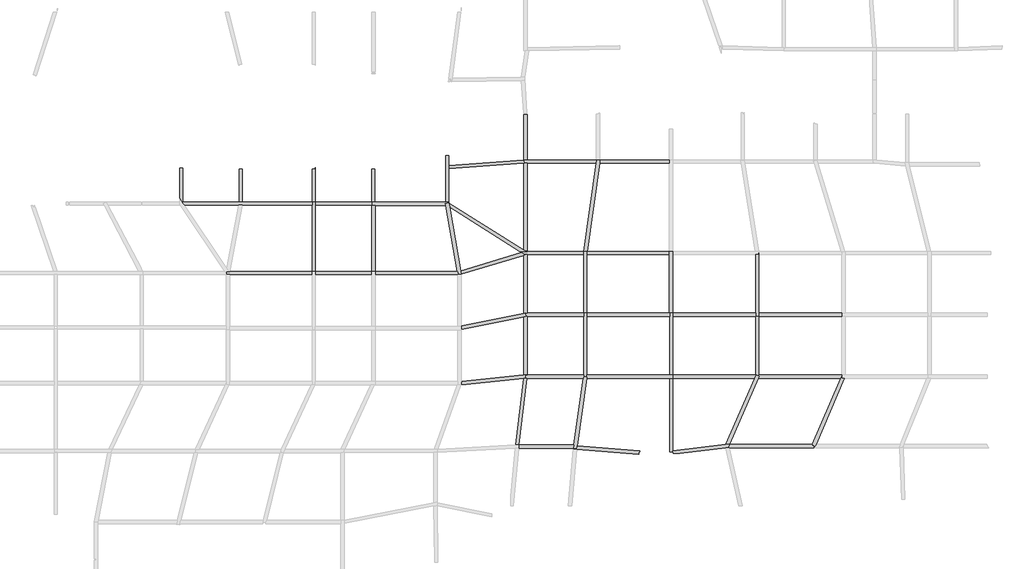
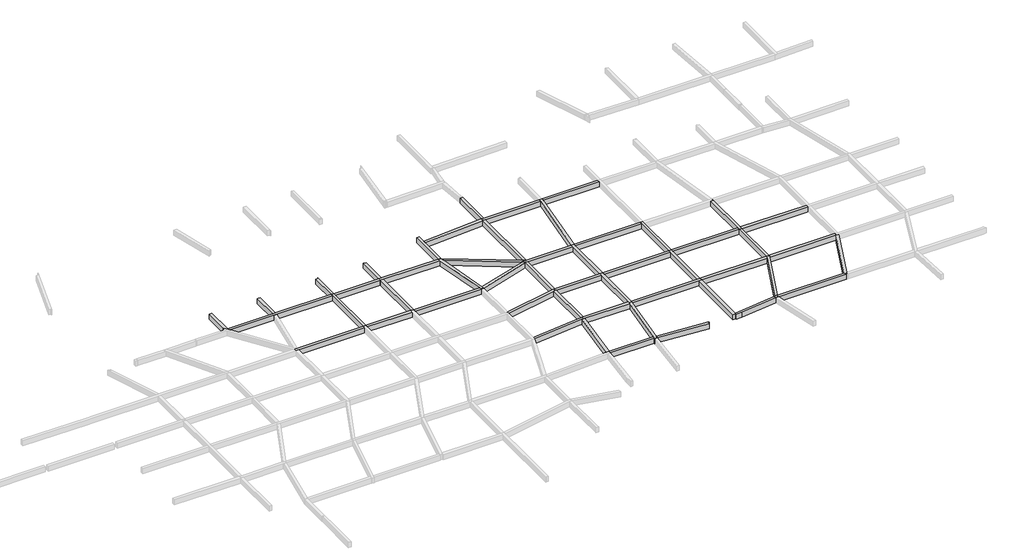
# One storey, part 10 of 15: 51 beams.
"""IFC4 building model written with IfcOpenShell, lengths in millimetres."""

from ifc_helpers import new_model, si_unit, frame, origin, place, context, project, spatial, polyline, outline, extrude, faceted_brep, element, save

model = new_model("IFC4")

# Units and contexts
model_context = context("Model", 3, world=origin())
ifc_project = project(units=[si_unit("LENGTHUNIT", "METRE", prefix="MILLI")], contexts=[model_context])

# Site, building, storey
site = spatial("IfcSite", under=ifc_project)
building = spatial("IfcBuilding", under=site)
storey = spatial("IfcBuildingStorey", under=building, Name="层高", Elevation=3300.0)

# Beams
placement = place(None, origin())
element("IfcBeam", 1, ObjectType="混凝土 - 矩形梁 : KL_beam", at=placement, inside=storey, context=model_context, shape_type="SweptSolid", body=[
    extrude(outline(polyline([(208450.3009381, 80084.9176514), (208450.3009381, 80384.9176514), (213550.3009381, 80384.9176514), (213550.3009381, 80084.9176514), (208450.3009381, 80084.9176514)])), frame((0.0, 0.0, 2700.0), z_axis=(0.0, 0.0, 1.0), x_axis=(1.0, 0.0, 0.0)), (0.0, 0.0, 1.0), 600.0),
])
element("IfcBeam", 2, ObjectType="混凝土 - 矩形梁 : KL_beam", at=placement, inside=storey, context=model_context, shape_type="Brep", body=[
    faceted_brep([(208150.3009381, 80092.1684205, 3300.0), (208150.3009381, 80384.9176514, 3300.0), (208450.3009381, 80384.9176514, 3300.0), (208450.3009381, 80392.1684205, 3300.0), (208150.3009381, 80392.1684205, 3300.0), (200691.8253203, 80392.1684205, 3300.0), (200590.9130323, 80392.1684205, 3300.0), (200361.325629, 80392.1684205, 3300.0), (200361.325629, 80196.1646357, 3300.0), (200361.325629, 80092.1684205, 3300.0), (200661.325629, 80092.1684205, 3300.0), (208150.3009381, 80092.1684205, 2700.0), (200361.325629, 80092.1684205, 2700.0), (200661.325629, 80092.1684205, 2700.0), (208150.3009381, 80384.9176514, 2700.0), (200361.325629, 80196.1646357, 2700.0), (200361.325629, 80392.1684205, 2700.0), (200590.9130323, 80392.1684205, 2700.0), (200691.8253203, 80392.1684205, 2700.0), (208150.3009381, 80392.1684205, 2700.0), (208450.3009381, 80392.1684205, 2700.0), (208450.3009381, 80384.9176514, 2700.0)], [[[0, 1, 2, 3, 4, 5, 6, 7, 8, 9, 10]], [[11, 0, 10, 9, 12, 13]], [[14, 11, 13, 12, 15, 16, 17, 18, 19, 20, 21]], [[16, 7, 6, 5, 4, 3, 20, 19, 18, 17]], [[14, 1, 0, 11]], [[1, 14, 21, 2]], [[9, 8, 7, 16, 15, 12]], [[20, 3, 2, 21]]]),
])
element("IfcBeam", 3, ObjectType="混凝土 - 矩形梁 : KL_beam", at=placement, inside=storey, context=model_context, shape_type="Brep", body=[
    faceted_brep([(232749.8021762, 70852.5016685, 3300.0), (233049.8021762, 70831.5236249, 3300.0), (233049.8021762, 70992.0126454, 3300.0), (233049.8021762, 76292.0126467, 3300.0), (233049.8021762, 76592.0126467, 3300.0), (232749.8021762, 76592.0126467, 3300.0), (232749.8021762, 76292.0126467, 3300.0), (232749.8021762, 70992.0126467, 3300.0), (233049.8021762, 70831.5236249, 2700.0), (233049.8021762, 70992.0126454, 2700.0), (233049.8021762, 76292.0126467, 2700.0), (233049.8021762, 76592.0126467, 2700.0), (232749.8021762, 70852.5016685, 2700.0), (232749.8021762, 70992.0126467, 2700.0), (232749.8021762, 76292.0126467, 2700.0), (232749.8021762, 76592.0126467, 2700.0)], [[[0, 1, 2, 3, 4, 5, 6, 7]], [[1, 8, 9, 10, 11, 4, 3, 2]], [[8, 12, 13, 14, 15, 11, 10, 9]], [[12, 0, 7, 6, 5, 15, 14, 13]], [[0, 12, 8, 1]], [[5, 4, 11, 15]]]),
])
element("IfcBeam", 4, ObjectType="混凝土 - 矩形梁 : KL_beam", at=placement, inside=storey, context=model_context, shape_type="Brep", body=[
    faceted_brep([(232124.0582724, 64244.513481, 3300.0), (232165.8855427, 64542.1299739, 3300.0), (233030.1951867, 70692.0126454, 3300.0), (233049.8021762, 70831.5236249, 3300.0), (232749.8021762, 70852.5016685, 3300.0), (232727.2469151, 70692.0126467, 3300.0), (231875.9120638, 64634.4504224, 3300.0), (231833.7498134, 64334.4504224, 3300.0), (231826.9778517, 64286.2654113, 3300.0), (232749.8021762, 70852.5016685, 2700.0), (232727.2469151, 70692.0126467, 2700.0), (231875.9120638, 64634.4504224, 2700.0), (231833.7498134, 64334.4504224, 2700.0), (231826.9778517, 64286.2654113, 2700.0), (233049.8021762, 70831.5236249, 2700.0), (233030.1951867, 70692.0126454, 2700.0), (232165.8855427, 64542.1299739, 2700.0), (232124.0582724, 64244.513481, 2700.0)], [[[0, 1, 2, 3, 4, 5, 6, 7, 8]], [[8, 7, 6, 5, 4, 9, 10, 11, 12, 13]], [[13, 12, 11, 10, 9, 14, 15, 16, 17]], [[3, 2, 1, 0, 17, 16, 15, 14]], [[3, 14, 9, 4]], [[0, 8, 13, 17]]]),
])
element("IfcBeam", 5, ObjectType="混凝土 - 矩形梁 : KL_beam", at=placement, inside=storey, context=model_context, shape_type="Brep", body=[
    faceted_brep([(233049.8021762, 70831.5236249, 3300.0), (233030.1951867, 70692.0126454, 3300.0), (240549.8021765, 70692.0126454, 3300.0), (240849.8021765, 70692.0126454, 3300.0), (240849.8021765, 70992.0126454, 3300.0), (240549.8021765, 70992.0126454, 3300.0), (233049.8021762, 70992.0126454, 3300.0), (240849.8021765, 70992.0126454, 2700.0), (240549.8021765, 70992.0126454, 2700.0), (233049.8021762, 70992.0126454, 2700.0), (233030.1951867, 70692.0126454, 2700.0), (233049.8021762, 70831.5236249, 2700.0), (240849.8021765, 70692.0126454, 2700.0), (240549.8021765, 70692.0126454, 2700.0)], [[[0, 1, 2, 3, 4, 5, 6]], [[4, 7, 8, 9, 6, 5]], [[10, 11, 9, 8, 7, 12, 13]], [[1, 10, 13, 12, 3, 2]], [[1, 0, 11, 10]], [[0, 6, 9, 11]], [[4, 3, 12, 7]]]),
])
element("IfcBeam", 6, ObjectType="混凝土 - 矩形梁 : KL_beam", at=placement, inside=storey, context=model_context, shape_type="Brep", body=[
    faceted_brep([(240849.8021765, 76592.0126467, 3300.0), (240838.5455997, 76592.0126467, 3300.0), (240549.8021765, 76592.0126467, 3300.0), (240549.8021765, 76292.0126467, 3300.0), (240549.8021765, 70992.0126454, 3300.0), (240849.8021765, 70992.0126454, 3300.0), (240849.8021765, 76302.5702379, 3300.0), (240849.8021765, 76592.0126467, 2700.0), (240849.8021765, 70992.0126454, 2700.0), (240849.8021765, 76302.5702379, 2700.0), (240549.8021765, 76592.0126467, 2700.0), (240838.5455997, 76592.0126467, 2700.0), (240549.8021765, 70992.0126454, 2700.0), (240549.8021765, 76292.0126467, 2700.0)], [[[0, 1, 2, 3, 4, 5, 6]], [[7, 0, 6, 5, 8, 9]], [[10, 11, 7, 9, 8, 12, 13]], [[2, 10, 13, 12, 4, 3]], [[5, 4, 12, 8]], [[2, 1, 0, 7, 11, 10]]]),
])
element("IfcBeam", 7, ObjectType="混凝土 - 矩形梁 : KL_beam", at=placement, inside=storey, context=model_context, shape_type="Brep", body=[
    faceted_brep([(233049.8021762, 76592.0126467, 3300.0), (233049.8021762, 76292.0126467, 3300.0), (240549.8021765, 76292.0126467, 3300.0), (240549.8021765, 76592.0126467, 3300.0), (240538.5455997, 76592.0126467, 3300.0), (233049.8021762, 76292.0126467, 2700.0), (240549.8021765, 76292.0126467, 2700.0), (233049.8021762, 76592.0126467, 2700.0), (240538.5455997, 76592.0126467, 2700.0), (240549.8021765, 76592.0126467, 2700.0)], [[[0, 1, 2, 3, 4]], [[1, 5, 6, 2]], [[5, 7, 8, 9, 6]], [[7, 0, 4, 3, 9, 8]], [[1, 0, 7, 5]], [[3, 2, 6, 9]]]),
])
element("IfcBeam", 8, ObjectType="混凝土 - 矩形梁 : KL_beam", at=placement, inside=storey, context=model_context, shape_type="Brep", body=[
    faceted_brep([(240849.8021765, 70692.0126454, 3300.0), (240549.8021765, 70692.0126454, 3300.0), (240549.8021765, 64002.26105, 3300.0), (240849.8021765, 64002.26105, 3300.0), (240849.8021765, 64111.1304578, 3300.0), (240549.8021765, 70692.0126454, 2700.0), (240549.8021765, 64002.26105, 2700.0), (240849.8021765, 70692.0126454, 2700.0), (240849.8021765, 64111.1304578, 2700.0), (240849.8021765, 64002.26105, 2700.0)], [[[0, 1, 2, 3, 4]], [[1, 5, 6, 2]], [[5, 7, 8, 9, 6]], [[7, 0, 4, 3, 9, 8]], [[1, 0, 7, 5]], [[3, 2, 6, 9]]]),
])
element("IfcBeam", 9, ObjectType="混凝土 - 矩形梁 : KL_beam", at=placement, inside=storey, context=model_context, shape_type="Brep", body=[
    faceted_brep([(245852.6551201, 64403.2000817, 3300.0), (245978.7341491, 64692.0126465, 3300.0), (245991.7500654, 64721.8285502, 3300.0), (245646.5106834, 64680.8252113, 3300.0), (240849.8021765, 64111.1304578, 3300.0), (240849.8021765, 64002.26105, 3300.0), (240859.8021767, 64002.26105, 3300.0), (240859.8021767, 63882.26105, 3300.0), (241466.459407, 63882.26105, 3300.0), (245632.7131892, 64377.0780516, 3300.0), (245758.4592979, 64392.0126465, 3300.0), (240849.8021765, 64111.1304578, 2700.0), (245991.7500654, 64721.8285502, 2700.0), (245646.5106834, 64680.8252113, 2700.0), (245978.7341491, 64692.0126465, 2700.0), (245852.6551201, 64403.2000817, 2700.0), (245758.4592979, 64392.0126465, 2700.0), (245632.7131892, 64377.0780516, 2700.0), (241466.459407, 63882.26105, 2700.0), (240859.8021767, 63882.26105, 2700.0), (240859.8021767, 64002.26105, 2700.0), (240849.8021765, 64002.26105, 2700.0)], [[[0, 1, 2, 3, 4, 5, 6, 7, 8, 9, 10]], [[11, 4, 3, 2, 12, 13]], [[12, 14, 15, 16, 17, 18, 19, 20, 21, 11, 13]], [[15, 0, 10, 9, 8, 18, 17, 16]], [[4, 11, 21, 5]], [[2, 1, 0, 15, 14, 12]], [[20, 6, 5, 21]], [[6, 20, 19, 7]], [[18, 8, 7, 19]]]),
])
element("IfcBeam", 10, ObjectType="混凝土 - 矩形梁 : KL_beam", at=placement, inside=storey, context=model_context, shape_type="Brep", body=[
    faceted_brep([(248676.5575109, 70871.9879428, 3300.0), (248649.8021768, 70883.6677897, 3300.0), (248401.6137516, 70992.0126454, 3300.0), (248270.650929, 70692.0126454, 3300.0), (245646.5106834, 64680.8252113, 3300.0), (245991.7500654, 64721.8285502, 3300.0), (248597.990601, 70692.0126454, 3300.0), (248401.6137516, 70992.0126454, 2700.0), (248270.650929, 70692.0126454, 2700.0), (245646.5106834, 64680.8252113, 2700.0), (248649.8021768, 70883.6677897, 2700.0), (248676.5575109, 70871.9879428, 2700.0), (248597.990601, 70692.0126454, 2700.0), (245991.7500654, 64721.8285502, 2700.0)], [[[0, 1, 2, 3, 4, 5, 6]], [[2, 7, 8, 9, 4, 3]], [[7, 10, 11, 12, 13, 9, 8]], [[11, 0, 6, 5, 13, 12]], [[5, 4, 9, 13]], [[0, 11, 10, 7, 2, 1]]]),
])
element("IfcBeam", 11, ObjectType="混凝土 - 矩形梁 : KL_beam", at=placement, inside=storey, context=model_context, shape_type="Brep", body=[
    faceted_brep([(248401.6137516, 70992.0126454, 3300.0), (248349.8021768, 70992.0126454, 3300.0), (240849.8021765, 70992.0126454, 3300.0), (240849.8021765, 70692.0126454, 3300.0), (248270.650929, 70692.0126454, 3300.0), (240849.8021765, 70692.0126454, 2700.0), (248270.650929, 70692.0126454, 2700.0), (240849.8021765, 70992.0126454, 2700.0), (248349.8021768, 70992.0126454, 2700.0), (248401.6137516, 70992.0126454, 2700.0)], [[[0, 1, 2, 3, 4]], [[3, 5, 6, 4]], [[7, 8, 9, 6, 5]], [[2, 1, 0, 9, 8, 7]], [[3, 2, 7, 5]], [[0, 4, 6, 9]]]),
])
element("IfcBeam", 12, ObjectType="混凝土 - 矩形梁 : KL_beam", at=placement, inside=storey, context=model_context, shape_type="Brep", body=[
    faceted_brep([(233049.8021762, 82197.4603606, 3300.0), (232769.4091655, 82197.4603606, 3300.0), (232749.8021762, 82197.4603606, 3300.0), (232749.8021762, 81897.4603606, 3300.0), (232749.8021762, 76592.0126467, 3300.0), (233049.8021762, 76592.0126467, 3300.0), (233049.8021762, 81897.4603606, 3300.0), (232749.8021762, 82197.4603606, 2700.0), (232749.8021762, 81897.4603606, 2700.0), (232749.8021762, 76592.0126467, 2700.0), (232769.4091655, 82197.4603606, 2700.0), (233049.8021762, 82197.4603606, 2700.0), (233049.8021762, 81897.4603606, 2700.0), (233049.8021762, 76592.0126467, 2700.0)], [[[0, 1, 2, 3, 4, 5, 6]], [[2, 7, 8, 9, 4, 3]], [[7, 10, 11, 12, 13, 9, 8]], [[11, 0, 6, 5, 13, 12]], [[5, 4, 9, 13]], [[2, 1, 0, 11, 10, 7]]]),
])
element("IfcBeam", 13, ObjectType="混凝土 - 矩形梁 : KL_beam", at=placement, inside=storey, context=model_context, shape_type="Brep", body=[
    faceted_brep([(240538.5455997, 76592.0126467, 3300.0), (240549.8021765, 76592.0126467, 3300.0), (240838.5455997, 76592.0126467, 3300.0), (240838.5455997, 76602.5702379, 3300.0), (240838.5455997, 81897.4603606, 3300.0), (240838.5455997, 82197.4603606, 3300.0), (240538.5455997, 82197.4603606, 3300.0), (240538.5455997, 81897.4603606, 3300.0), (240538.5455997, 82197.4603606, 2700.0), (240538.5455997, 81897.4603606, 2700.0), (240538.5455997, 76592.0126467, 2700.0), (240838.5455997, 76592.0126467, 2700.0), (240549.8021765, 76592.0126467, 2700.0), (240838.5455997, 82197.4603606, 2700.0), (240838.5455997, 81897.4603606, 2700.0), (240838.5455997, 76602.5702379, 2700.0)], [[[0, 1, 2, 3, 4, 5, 6, 7]], [[6, 8, 9, 10, 0, 7]], [[11, 12, 10, 9, 8, 13, 14, 15]], [[2, 11, 15, 14, 13, 5, 4, 3]], [[0, 10, 12, 11, 2, 1]], [[6, 5, 13, 8]]]),
])
element("IfcBeam", 14, ObjectType="混凝土 - 矩形梁 : KL_beam", at=placement, inside=storey, context=model_context, shape_type="Brep", body=[
    faceted_brep([(233049.8021762, 82197.4603606, 3300.0), (233049.8021762, 81897.4603606, 3300.0), (240538.5455997, 81897.4603606, 3300.0), (240538.5455997, 82197.4603606, 3300.0), (233072.3574373, 82197.4603606, 3300.0), (233049.8021762, 81897.4603606, 2700.0), (240538.5455997, 81897.4603606, 2700.0), (233049.8021762, 82197.4603606, 2700.0), (233072.3574373, 82197.4603606, 2700.0), (240538.5455997, 82197.4603606, 2700.0)], [[[0, 1, 2, 3, 4]], [[1, 5, 6, 2]], [[5, 7, 8, 9, 6]], [[7, 0, 4, 3, 9, 8]], [[1, 0, 7, 5]], [[3, 2, 6, 9]]]),
])
element("IfcBeam", 15, ObjectType="混凝土 - 矩形梁 : KL_beam", at=placement, inside=storey, context=model_context, shape_type="Brep", body=[
    faceted_brep([(232749.8021762, 81897.4603606, 3300.0), (232749.8021762, 82197.4603606, 3300.0), (227629.4690157, 82197.4603606, 3300.0), (227522.8372624, 82197.4603606, 3300.0), (226960.6562509, 82197.4603606, 3300.0), (227121.3961295, 82096.0353536, 3300.0), (227436.1007689, 81897.4603606, 3300.0), (227501.6199656, 81897.4603606, 3300.0), (227629.4690157, 81897.4603606, 3300.0), (232749.8021762, 82197.4603606, 2700.0), (227629.4690157, 82197.4603606, 2700.0), (227522.8372624, 82197.4603606, 2700.0), (226960.6562509, 82197.4603606, 2700.0), (232749.8021762, 81897.4603606, 2700.0), (227629.4690157, 81897.4603606, 2700.0), (227501.6199656, 81897.4603606, 2700.0), (227436.1007689, 81897.4603606, 2700.0), (227121.3961295, 82096.0353536, 2700.0)], [[[0, 1, 2, 3, 4, 5, 6, 7, 8]], [[1, 9, 10, 11, 12, 4, 3, 2]], [[9, 13, 14, 15, 16, 17, 12, 11, 10]], [[13, 0, 8, 7, 6, 16, 15, 14]], [[1, 0, 13, 9]], [[6, 5, 4, 12, 17, 16]]]),
])
element("IfcBeam", 16, ObjectType="混凝土 - 矩形梁 : KL_beam", at=placement, inside=storey, context=model_context, shape_type="Brep", body=[
    faceted_brep([(227464.5672467, 76592.0126467, 3300.0), (227494.3707847, 76292.0126467, 3300.0), (227629.4690157, 76292.0126467, 3300.0), (232749.8021762, 76292.0126467, 3300.0), (232749.8021762, 76592.0126467, 3300.0), (227629.4690157, 76592.0126467, 3300.0), (227464.5672467, 76592.0126467, 2700.0), (232749.8021762, 76592.0126467, 2700.0), (227629.4690157, 76592.0126467, 2700.0), (227494.3707847, 76292.0126467, 2700.0), (232749.8021762, 76292.0126467, 2700.0), (227629.4690157, 76292.0126467, 2700.0)], [[[0, 1, 2, 3, 4, 5]], [[6, 0, 5, 4, 7, 8]], [[9, 6, 8, 7, 10, 11]], [[1, 9, 11, 10, 3, 2]], [[4, 3, 10, 7]], [[1, 0, 6, 9]]]),
])
element("IfcBeam", 17, ObjectType="混凝土 - 矩形梁 : KL_beam", at=placement, inside=storey, context=model_context, shape_type="Brep", body=[
    faceted_brep([(232749.8021762, 70992.0126467, 3300.0), (227648.3553452, 70992.0126467, 3300.0), (227471.9636762, 70992.0126467, 3300.0), (227486.9743551, 70692.0126467, 3300.0), (227612.6947188, 70692.0126467, 3300.0), (232727.2469151, 70692.0126467, 3300.0), (232749.8021762, 70852.5016685, 3300.0), (232749.8021762, 70992.0126467, 2700.0), (227648.3553452, 70992.0126467, 2700.0), (227471.9636762, 70992.0126467, 2700.0), (232749.8021762, 70852.5016685, 2700.0), (232727.2469151, 70692.0126467, 2700.0), (227612.6947188, 70692.0126467, 2700.0), (227486.9743551, 70692.0126467, 2700.0)], [[[0, 1, 2, 3, 4, 5, 6]], [[2, 1, 0, 7, 8, 9]], [[9, 8, 7, 10, 11, 12, 13]], [[3, 13, 12, 11, 5, 4]], [[0, 6, 10, 7]], [[6, 5, 11, 10]], [[3, 2, 9, 13]]]),
])
element("IfcBeam", 18, ObjectType="混凝土 - 矩形梁 : KL_beam", at=placement, inside=storey, context=model_context, shape_type="Brep", body=[
    faceted_brep([(220529.7964704, 86609.9883385, 3300.0), (220234.3541445, 86557.8938852, 3300.0), (220267.7389156, 86368.5594398, 3300.0), (221321.5378995, 80392.1684205, 3300.0), (221374.4359938, 80092.1684205, 3300.0), (221375.7053189, 80084.9697198, 3300.0), (221416.5311794, 80092.1684205, 3300.0), (221650.3009384, 80133.3883363, 3300.0), (221671.1476448, 80137.0641731, 3300.0), (221618.6840658, 80434.599915, 3300.0), (220600.1752559, 86210.850412, 3300.0), (220529.7964704, 86609.9883385, 2700.0), (221671.1476448, 80137.0641731, 2700.0), (221618.6840658, 80434.599915, 2700.0), (220600.1752559, 86210.850412, 2700.0), (220234.3541445, 86557.8938852, 2700.0), (221650.3009384, 80133.3883363, 2700.0), (221416.5311794, 80092.1684205, 2700.0), (221375.7053189, 80084.9697198, 2700.0), (221374.4359938, 80092.1684205, 2700.0), (221321.5378995, 80392.1684205, 2700.0), (220267.7389156, 86368.5594398, 2700.0)], [[[0, 1, 2, 3, 4, 5, 6, 7, 8, 9, 10]], [[11, 0, 10, 9, 8, 12, 13, 14]], [[15, 11, 14, 13, 12, 16, 17, 18, 19, 20, 21]], [[1, 15, 21, 20, 19, 18, 5, 4, 3, 2]], [[1, 0, 11, 15]], [[5, 18, 17, 16, 12, 8, 7, 6]]]),
])
element("IfcBeam", 19, ObjectType="混凝土 - 矩形梁 : KL_beam", at=placement, inside=storey, context=model_context, shape_type="Brep", body=[
    faceted_brep([(227522.8372624, 82197.4603606, 3300.0), (227501.6325968, 82210.8402598, 3300.0), (227329.4690157, 82319.4734911, 3300.0), (220543.6038603, 86601.2760349, 3300.0), (220529.7964704, 86609.9883385, 3300.0), (220600.1752559, 86210.850412, 3300.0), (226960.6562509, 82197.4603606, 3300.0), (226960.6562509, 82197.4603606, 2700.0), (220600.1752559, 86210.850412, 2700.0), (220529.7964704, 86609.9883385, 2700.0), (220543.6038603, 86601.2760349, 2700.0), (227329.4690157, 82319.4734911, 2700.0), (227501.6325968, 82210.8402598, 2700.0), (227522.8372624, 82197.4603606, 2700.0)], [[[0, 1, 2, 3, 4, 5, 6]], [[7, 6, 5, 8]], [[9, 10, 11, 12, 13, 7, 8]], [[4, 3, 2, 1, 0, 13, 12, 11, 10, 9]], [[0, 6, 7, 13]], [[5, 4, 9, 8]]]),
])
element("IfcBeam", 20, ObjectType="混凝土 - 矩形梁 : KL_beam", at=placement, inside=storey, context=model_context, shape_type="Brep", body=[
    faceted_brep([(227501.6325968, 82210.8402598, 3300.0), (227522.8372624, 82197.4603606, 3300.0), (227629.4690157, 82197.4603606, 3300.0), (227629.4690157, 82249.4379465, 3300.0), (227522.8372624, 82197.4603606, 2700.0), (227501.6325968, 82210.8402598, 2700.0), (227629.4690157, 82249.4379465, 2700.0), (227629.4690157, 82197.4603606, 2700.0)], [[[0, 1, 2, 3]], [[4, 5, 6, 7]], [[5, 0, 3, 6]], [[1, 4, 7, 2]], [[1, 0, 5, 4]], [[6, 3, 2, 7]]]),
    faceted_brep([(227501.6199656, 81897.4603606, 3300.0), (227329.4690157, 81845.4827747, 3300.0), (221671.1476448, 80137.0641731, 3300.0), (221671.1476448, 80137.0641731, 2700.0), (227329.4690157, 81845.4827747, 2700.0), (227501.6199656, 81897.4603606, 2700.0), (227436.1007689, 81897.4603606, 2700.0), (227436.1007689, 81897.4603606, 3300.0), (227121.3961295, 82096.0353536, 2700.0), (227121.3961295, 82096.0353536, 3300.0), (221618.6840658, 80434.599915, 3300.0), (221618.6840658, 80434.599915, 2700.0)], [[[0, 1, 2, 3, 4, 5]], [[6, 7, 0, 5]], [[7, 6, 8, 9]], [[2, 1, 0, 7, 9, 10]], [[5, 4, 3, 11, 8, 6]], [[9, 8, 11, 10]], [[3, 2, 10, 11]]]),
])
element("IfcBeam", 21, ObjectType="混凝土 - 矩形梁 : KL_beam", at=placement, inside=storey, context=model_context, shape_type="Brep", body=[
    faceted_brep([(213550.3009381, 80392.1684205, 3300.0), (213550.3009381, 80384.9176514, 3300.0), (213850.3009381, 80384.9176514, 3300.0), (213850.3009381, 80092.1684205, 3300.0), (221350.3009384, 80092.1684205, 3300.0), (221374.4359938, 80092.1684205, 3300.0), (221329.454232, 80347.2726679, 3300.0), (221321.5378995, 80392.1684205, 3300.0), (213850.3009381, 80392.1684205, 3300.0), (213550.3009381, 80392.1684205, 2700.0), (221321.5378995, 80392.1684205, 2700.0), (213850.3009381, 80392.1684205, 2700.0), (213550.3009381, 80384.9176514, 2700.0), (221329.454232, 80347.2726679, 2700.0), (221374.4359938, 80092.1684205, 2700.0), (221350.3009384, 80092.1684205, 2700.0), (213850.3009381, 80092.1684205, 2700.0), (213850.3009381, 80384.9176514, 2700.0)], [[[0, 1, 2, 3, 4, 5, 6, 7, 8]], [[9, 0, 8, 7, 10, 11]], [[12, 9, 11, 10, 13, 14, 15, 16, 17]], [[3, 16, 15, 14, 5, 4]], [[0, 9, 12, 1]], [[2, 17, 16, 3]], [[17, 2, 1, 12]], [[10, 7, 6, 5, 14, 13]]]),
    faceted_brep([(221416.5311794, 80092.1684205, 3300.0), (221650.3009384, 80133.3883363, 3300.0), (221650.3009384, 80133.3883363, 2700.0), (221416.5311794, 80092.1684205, 2700.0), (221650.3009384, 80092.1684205, 3300.0), (221650.3009384, 80092.1684205, 2700.0)], [[[0, 1, 2, 3]], [[4, 5, 2, 1]], [[1, 0, 4]], [[3, 2, 5]], [[0, 3, 5, 4]]]),
])
element("IfcBeam", 22, ObjectType="混凝土 - 矩形梁 : KL_beam", at=placement, inside=storey, context=model_context, shape_type="Brep", body=[
    faceted_brep([(208450.3009381, 86681.1826239, 3300.0), (208150.3009381, 86681.1826239, 3300.0), (208150.3009381, 86381.1826239, 3300.0), (208150.3009381, 80392.1684205, 3300.0), (208450.3009381, 80392.1684205, 3300.0), (208450.3009381, 86381.1826239, 3300.0), (208450.3009381, 86681.1826239, 2700.0), (208450.3009381, 80392.1684205, 2700.0), (208450.3009381, 86381.1826239, 2700.0), (208150.3009381, 86681.1826239, 2700.0), (208150.3009381, 80392.1684205, 2700.0), (208150.3009381, 86381.1826239, 2700.0)], [[[0, 1, 2, 3, 4, 5]], [[6, 0, 5, 4, 7, 8]], [[9, 6, 8, 7, 10, 11]], [[1, 9, 11, 10, 3, 2]], [[4, 3, 10, 7]], [[1, 0, 6, 9]]]),
])
element("IfcBeam", 23, ObjectType="混凝土 - 矩形梁 : KL_beam", at=placement, inside=storey, context=model_context, shape_type="Brep", body=[
    faceted_brep([(213543.6038603, 86668.5594398, 3300.0), (213543.6038603, 86381.1826239, 3300.0), (213543.6038603, 86368.5594398, 3300.0), (213550.3009381, 86368.5594398, 3300.0), (213850.3009381, 86368.5594398, 3300.0), (220267.7389156, 86368.5594398, 3300.0), (220257.4112501, 86427.130541, 3300.0), (220234.3541445, 86557.8938852, 3300.0), (220529.7964704, 86609.9883385, 3300.0), (220543.6038603, 86601.2760349, 3300.0), (220543.6038603, 86668.5594398, 3300.0), (220243.6038603, 86668.5594398, 3300.0), (213843.6038603, 86668.5594398, 3300.0), (213543.6038603, 86668.5594398, 2700.0), (220543.6038603, 86668.5594398, 2700.0), (220243.6038603, 86668.5594398, 2700.0), (213843.6038603, 86668.5594398, 2700.0), (213543.6038603, 86368.5594398, 2700.0), (213543.6038603, 86381.1826239, 2700.0), (220543.6038603, 86601.2760349, 2700.0), (220529.7964704, 86609.9883385, 2700.0), (220234.3541445, 86557.8938852, 2700.0), (220257.4112501, 86427.130541, 2700.0), (220267.7389156, 86368.5594398, 2700.0), (213850.3009381, 86368.5594398, 2700.0), (213550.3009381, 86368.5594398, 2700.0)], [[[0, 1, 2, 3, 4, 5, 6, 7, 8, 9, 10, 11, 12]], [[13, 0, 12, 11, 10, 14, 15, 16]], [[17, 18, 13, 16, 15, 14, 19, 20, 21, 22, 23, 24, 25]], [[23, 5, 4, 3, 2, 17, 25, 24]], [[5, 23, 22, 21, 7, 6]], [[2, 1, 0, 13, 18, 17]], [[14, 10, 9, 19]], [[7, 21, 20, 8]], [[9, 8, 20, 19]]]),
])
element("IfcBeam", 24, ObjectType="混凝土 - 矩形梁 : KL_beam", at=placement, inside=storey, context=model_context, shape_type="Brep", body=[
    faceted_brep([(196128.3344611, 89741.5754183, 3300.0), (196428.3344611, 89741.5754183, 3300.0), (196428.3344611, 89741.5754183, 2700.0), (196128.3344611, 89741.5754183, 2700.0), (196128.3344611, 86983.1947852, 3300.0), (196428.3344611, 86540.1083772, 3300.0), (196428.3344611, 86681.1826239, 3300.0), (196428.3344611, 86540.1083772, 2700.0), (196428.3344611, 86681.1826239, 2700.0), (196128.3344611, 86983.1947852, 2700.0)], [[[0, 1, 2, 3]], [[1, 0, 4, 5, 6]], [[2, 1, 6, 5, 7, 8]], [[3, 2, 8, 7, 9]], [[0, 3, 9, 4]], [[5, 4, 9, 7]]]),
])
element("IfcBeam", 25, ObjectType="混凝土 - 矩形梁 : KL_beam", at=placement, inside=storey, context=model_context, shape_type="Brep", body=[
    faceted_brep([(253461.7702502, 64601.2338843, 3300.0), (253461.7702502, 64601.2338843, 2700.0), (253599.5848532, 64542.165729, 2700.0), (253689.5875713, 64503.5900308, 2700.0), (253689.5875713, 64503.5900308, 3300.0), (253599.5848532, 64542.165729, 3300.0), (256398.7084648, 70692.0126466, 3300.0), (256149.8021771, 70692.0126466, 3300.0), (256149.8021771, 70872.8035797, 3300.0), (256072.3141117, 70692.0126454, 3300.0), (253500.6785655, 64692.0126465, 3300.0), (253689.5875713, 64542.2610502, 3300.0), (253762.8884968, 64542.2610502, 3300.0), (253827.0729182, 64692.0126466, 3300.0), (256398.7084648, 70692.0126466, 2700.0), (253762.8884968, 64542.2610502, 2700.0), (253827.0729182, 64692.0126466, 2700.0), (256149.8021771, 70692.0126466, 2700.0), (253689.5875713, 64542.2610502, 2700.0), (253500.6785655, 64692.0126465, 2700.0), (256072.3141117, 70692.0126454, 2700.0), (256149.8021771, 70872.8035797, 2700.0)], [[[0, 1, 2, 3, 4, 5]], [[6, 7, 8, 9, 10, 0, 5, 4, 11, 12, 13]], [[14, 6, 13, 12, 15, 16]], [[17, 14, 16, 15, 18, 3, 2, 1, 19, 20, 21]], [[1, 0, 10, 9, 8, 21, 20, 19]], [[17, 7, 6, 14]], [[7, 17, 21, 8]], [[18, 11, 4, 3]], [[11, 18, 15, 12]]]),
])
element("IfcBeam", 26, ObjectType="混凝土 - 矩形梁 : KL_beam", at=placement, inside=storey, context=model_context, shape_type="Brep", body=[
    faceted_brep([(208150.3009381, 86381.1826239, 3300.0), (208150.3009381, 86681.1826239, 3300.0), (201832.0411038, 86681.1826239, 3300.0), (201532.0411038, 86681.1826239, 3300.0), (196428.3344611, 86681.1826239, 3300.0), (196428.3344611, 86540.1083772, 3300.0), (196535.9381364, 86381.1826239, 3300.0), (201501.5414125, 86381.1826239, 3300.0), (201806.6950566, 86381.1826239, 3300.0), (208150.3009381, 86381.1826239, 2700.0), (196535.9381364, 86381.1826239, 2700.0), (201501.5414125, 86381.1826239, 2700.0), (201806.6950566, 86381.1826239, 2700.0), (208150.3009381, 86681.1826239, 2700.0), (196428.3344611, 86540.1083772, 2700.0), (196428.3344611, 86681.1826239, 2700.0), (201532.0411038, 86681.1826239, 2700.0), (201832.0411038, 86681.1826239, 2700.0)], [[[0, 1, 2, 3, 4, 5, 6, 7, 8]], [[9, 0, 8, 7, 6, 10, 11, 12]], [[13, 9, 12, 11, 10, 14, 15, 16, 17]], [[1, 13, 17, 16, 15, 4, 3, 2]], [[1, 0, 9, 13]], [[4, 15, 14, 5]], [[6, 5, 14, 10]]]),
])
element("IfcBeam", 27, ObjectType="混凝土 - 矩形梁 : KL_beam", at=placement, inside=storey, context=model_context, shape_type="Brep", body=[
    faceted_brep([(208450.3009381, 86681.1826239, 3300.0), (208450.3009381, 86381.1826239, 3300.0), (213543.6038603, 86381.1826239, 3300.0), (213543.6038603, 86668.5594398, 3300.0), (213543.6038603, 86681.1826239, 3300.0), (208450.3009381, 86381.1826239, 2700.0), (213543.6038603, 86381.1826239, 2700.0), (208450.3009381, 86681.1826239, 2700.0), (213543.6038603, 86681.1826239, 2700.0), (213543.6038603, 86668.5594398, 2700.0)], [[[0, 1, 2, 3, 4]], [[1, 5, 6, 2]], [[5, 7, 8, 9, 6]], [[7, 0, 4, 8]], [[1, 0, 7, 5]], [[2, 6, 9, 8, 4, 3]]]),
])
element("IfcBeam", 28, ObjectType="混凝土 - 矩形梁 : KL_beam", at=placement, inside=storey, context=model_context, shape_type="SweptSolid", body=[
    extrude(outline(polyline([(208450.3009381, 86681.1826239), (208150.3009381, 86681.1826239), (208150.3009381, 89682.0439941), (208449.2467743, 89682.0439941), (208449.2467743, 89802.0439941), (208450.3009381, 89802.0439941), (208450.3009381, 86681.1826239)])), frame((0.0, 0.0, 2700.0), z_axis=(0.0, 0.0, 1.0), x_axis=(1.0, 0.0, 0.0)), (0.0, 0.0, 1.0), 600.0),
])
element("IfcBeam", 29, ObjectType="混凝土 - 矩形梁 : KL_beam", at=placement, inside=storey, context=model_context, shape_type="Brep", body=[
    faceted_brep([(213543.6038603, 86668.5594398, 3300.0), (213843.6038603, 86668.5594398, 3300.0), (213843.6038603, 89682.0439941, 3300.0), (213649.2467743, 89682.0439941, 3300.0), (213543.6038603, 89682.0439941, 3300.0), (213543.6038603, 86681.1826239, 3300.0), (213843.6038603, 86668.5594398, 2700.0), (213843.6038603, 89682.0439941, 2700.0), (213543.6038603, 86668.5594398, 2700.0), (213543.6038603, 86681.1826239, 2700.0), (213543.6038603, 89682.0439941, 2700.0)], [[[0, 1, 2, 3, 4, 5]], [[1, 6, 7, 2]], [[6, 8, 9, 10, 7]], [[8, 0, 5, 4, 10, 9]], [[1, 0, 8, 6]], [[2, 7, 10, 4, 3]]]),
])
element("IfcBeam", 30, ObjectType="混凝土 - 矩形梁 : KL_beam", at=placement, inside=storey, context=model_context, shape_type="Brep", body=[
    faceted_brep([(201532.0411038, 86681.1826239, 3300.0), (201832.0411038, 86681.1826239, 3300.0), (201832.0411038, 89682.0439941, 3300.0), (201649.2467743, 89682.0439941, 3300.0), (201532.0411038, 89682.0439941, 3300.0), (201832.0411038, 86681.1826239, 2700.0), (201832.0411038, 89682.0439941, 2700.0), (201532.0411038, 86681.1826239, 2700.0), (201532.0411038, 89682.0439941, 2700.0)], [[[0, 1, 2, 3, 4]], [[1, 5, 6, 2]], [[5, 7, 8, 6]], [[7, 0, 4, 8]], [[1, 0, 7, 5]], [[2, 6, 8, 4, 3]]]),
])
element("IfcBeam", 31, ObjectType="混凝土 - 矩形梁 : KL_beam", at=placement, inside=storey, context=model_context, shape_type="Brep", body=[
    faceted_brep([(220243.6038603, 86668.5594398, 3300.0), (220543.6038603, 86668.5594398, 3300.0), (220543.6038603, 89691.9482279, 3300.0), (220543.6038603, 89992.7557999, 3300.0), (220543.6038603, 90882.0439942, 3300.0), (220243.6038603, 90882.0439942, 3300.0), (220543.6038603, 86668.5594398, 2700.0), (220543.6038603, 89691.9482279, 2700.0), (220543.6038603, 89992.7557999, 2700.0), (220543.6038603, 90882.0439942, 2700.0), (220243.6038603, 86668.5594398, 2700.0), (220243.6038603, 90882.0439942, 2700.0)], [[[0, 1, 2, 3, 4, 5]], [[1, 6, 7, 8, 9, 4, 3, 2]], [[6, 10, 11, 9, 8, 7]], [[10, 0, 5, 11]], [[1, 0, 10, 6]], [[5, 4, 9, 11]]]),
])
element("IfcBeam", 32, ObjectType="混凝土 - 矩形梁 : KL_beam", at=placement, inside=storey, context=model_context, shape_type="Brep", body=[
    faceted_brep([(232769.4091655, 82197.4603606, 3300.0), (233049.8021762, 82197.4603606, 3300.0), (233072.3574373, 82197.4603606, 3300.0), (234195.9034071, 90191.9053361, 3300.0), (234238.0656575, 90491.9053361, 3300.0), (234215.5103964, 90491.9053361, 3300.0), (233935.1173858, 90491.9053361, 3300.0), (233892.9551353, 90191.9053361, 3300.0), (233072.3574373, 82197.4603606, 2700.0), (234195.9034071, 90191.9053361, 2700.0), (234238.0656575, 90491.9053361, 2700.0), (233049.8021762, 82197.4603606, 2700.0), (232769.4091655, 82197.4603606, 2700.0), (233892.9551353, 90191.9053361, 2700.0), (233935.1173858, 90491.9053361, 2700.0), (234215.5103964, 90491.9053361, 2700.0)], [[[0, 1, 2, 3, 4, 5, 6, 7]], [[2, 8, 9, 10, 4, 3]], [[8, 11, 12, 13, 14, 15, 10, 9]], [[12, 0, 7, 6, 14, 13]], [[0, 12, 11, 8, 2, 1]], [[6, 5, 4, 10, 15, 14]]]),
])
element("IfcBeam", 33, ObjectType="混凝土 - 矩形梁 : KL_beam", at=placement, inside=storey, context=model_context, shape_type="Brep", body=[
    faceted_brep([(248649.8021768, 82041.877209, 3300.0), (248649.8021768, 82041.877209, 2700.0), (248627.0786147, 82041.877209, 2700.0), (248627.0786147, 82041.877209, 3300.0), (248649.8021768, 76302.5702379, 3300.0), (248649.8021768, 76602.5702379, 3300.0), (248649.8021768, 81897.4603606, 3300.0), (248627.0786147, 81897.4603606, 3300.0), (248349.8021768, 81897.4603606, 3300.0), (248349.8021768, 76602.5702379, 3300.0), (248349.8021768, 76302.5702379, 3300.0), (248649.8021768, 76302.5702379, 2700.0), (248649.8021768, 76602.5702379, 2700.0), (248649.8021768, 81897.4603606, 2700.0), (248349.8021768, 76302.5702379, 2700.0), (248349.8021768, 76602.5702379, 2700.0), (248349.8021768, 81897.4603606, 2700.0), (248627.0786147, 81897.4603606, 2700.0)], [[[0, 1, 2, 3]], [[4, 5, 6, 0, 3, 7, 8, 9, 10]], [[1, 0, 6, 5, 4, 11, 12, 13]], [[1, 13, 12, 11, 14, 15, 16, 17, 2]], [[14, 10, 9, 8, 16, 15]], [[7, 17, 16, 8]], [[17, 7, 3, 2]], [[4, 10, 14, 11]]]),
])
element("IfcBeam", 34, ObjectType="混凝土 - 矩形梁 : KL_beam", at=placement, inside=storey, context=model_context, shape_type="Brep", body=[
    faceted_brep([(248401.6137516, 70992.0126454, 3300.0), (248649.8021768, 70883.6677897, 3300.0), (248649.8021768, 70992.0126454, 3300.0), (248649.8021768, 76302.5702379, 3300.0), (248349.8021768, 76302.5702379, 3300.0), (248349.8021768, 70992.0126454, 3300.0), (248349.8021768, 76302.5702379, 2700.0), (248349.8021768, 70992.0126454, 2700.0), (248649.8021768, 70883.6677897, 2700.0), (248401.6137516, 70992.0126454, 2700.0), (248649.8021768, 76302.5702379, 2700.0), (248649.8021768, 70992.0126454, 2700.0)], [[[0, 1, 2, 3, 4, 5]], [[4, 6, 7, 5]], [[8, 9, 7, 6, 10, 11]], [[1, 8, 11, 10, 3, 2]], [[1, 0, 9, 8]], [[0, 5, 7, 9]], [[4, 3, 10, 6]]]),
])
element("IfcBeam", 35, ObjectType="混凝土 - 矩形梁 : KL_beam", at=placement, inside=storey, context=model_context, shape_type="SweptSolid", body=[
    extrude(outline(polyline([(240849.8021765, 76302.5702379), (240849.8021765, 76592.0126467), (240838.5455997, 76592.0126467), (240838.5455997, 76602.5702379), (248349.8021768, 76602.5702379), (248349.8021768, 76302.5702379), (240849.8021765, 76302.5702379)])), frame((0.0, 0.0, 2700.0), z_axis=(0.0, 0.0, 1.0), x_axis=(1.0, 0.0, 0.0)), (0.0, 0.0, 1.0), 600.0),
])
element("IfcBeam", 36, ObjectType="混凝土 - 矩形梁 : KL_beam", at=placement, inside=storey, context=model_context, shape_type="Brep", body=[
    faceted_brep([(256149.8021771, 76302.5702379, 3300.0), (256149.8021771, 76592.0126466, 3300.0), (256149.8021771, 76602.5702379, 3300.0), (248649.8021768, 76602.5702379, 3300.0), (248649.8021768, 76302.5702379, 3300.0), (256149.8021771, 76302.5702379, 2700.0), (248649.8021768, 76302.5702379, 2700.0), (256149.8021771, 76602.5702379, 2700.0), (256149.8021771, 76592.0126466, 2700.0), (248649.8021768, 76602.5702379, 2700.0)], [[[0, 1, 2, 3, 4]], [[5, 0, 4, 6]], [[7, 8, 5, 6, 9]], [[2, 7, 9, 3]], [[0, 5, 8, 7, 2, 1]], [[4, 3, 9, 6]]]),
])
element("IfcBeam", 37, ObjectType="混凝土 - 矩形梁 : KL_beam", at=placement, inside=storey, context=model_context, shape_type="SweptSolid", body=[
    extrude(outline(polyline([(240538.5455997, 90491.9053361), (240538.5455997, 90191.9053361), (234195.9034071, 90191.9053361), (234238.0656575, 90491.9053361), (240538.5455997, 90491.9053361)])), frame((0.0, 0.0, 2700.0), z_axis=(0.0, 0.0, 1.0), x_axis=(1.0, 0.0, 0.0)), (0.0, 0.0, 1.0), 600.0),
])
element("IfcBeam", 38, ObjectType="混凝土 - 矩形梁 : KL_beam", at=placement, inside=storey, context=model_context, shape_type="Brep", body=[
    faceted_brep([(227352.7974455, 90191.9053361, 3300.0), (227629.4690157, 90191.9053361, 3300.0), (233892.9551353, 90191.9053361, 3300.0), (233935.1173858, 90491.9053361, 3300.0), (233915.5103964, 90491.9053361, 3300.0), (227629.4690157, 90491.9053361, 3300.0), (227341.798674, 90491.9053361, 3300.0), (233935.1173858, 90491.9053361, 2700.0), (233915.5103964, 90491.9053361, 2700.0), (227629.4690157, 90491.9053361, 2700.0), (227341.798674, 90491.9053361, 2700.0), (233892.9551353, 90191.9053361, 2700.0), (227629.4690157, 90191.9053361, 2700.0), (227352.7974455, 90191.9053361, 2700.0)], [[[0, 1, 2, 3, 4, 5, 6]], [[6, 5, 4, 3, 7, 8, 9, 10]], [[10, 9, 8, 7, 11, 12, 13]], [[2, 1, 0, 13, 12, 11]], [[3, 2, 11, 7]], [[0, 6, 10, 13]]]),
])
element("IfcBeam", 39, ObjectType="混凝土 - 矩形梁 : KL_beam", at=placement, inside=storey, context=model_context, shape_type="Brep", body=[
    faceted_brep([(227352.7974455, 90191.9053361, 3300.0), (227341.798674, 90491.9053361, 3300.0), (227329.4690157, 90491.0000453, 3300.0), (220543.6038603, 89992.7557999, 3300.0), (220543.6038603, 89691.9482279, 3300.0), (227329.4690157, 90190.1924734, 3300.0), (227341.798674, 90491.9053361, 2700.0), (227329.4690157, 90491.0000453, 2700.0), (220543.6038603, 89992.7557999, 2700.0), (227352.7974455, 90191.9053361, 2700.0), (227329.4690157, 90190.1924734, 2700.0), (220543.6038603, 89691.9482279, 2700.0)], [[[0, 1, 2, 3, 4, 5]], [[1, 6, 7, 8, 3, 2]], [[6, 9, 10, 11, 8, 7]], [[9, 0, 5, 4, 11, 10]], [[0, 9, 6, 1]], [[4, 3, 8, 11]]]),
])
element("IfcBeam", 40, ObjectType="混凝土 - 矩形梁 : KL_beam", at=placement, inside=storey, context=model_context, shape_type="SweptSolid", body=[
    extrude(outline(polyline([(227501.6325968, 82210.8402598), (227329.4690157, 82319.4734911), (227329.4690157, 90190.1924734), (227352.7974455, 90191.9053361), (227629.4690157, 90191.9053361), (227629.4690157, 82249.4379465), (227501.6325968, 82210.8402598)])), frame((0.0, 0.0, 2700.0), z_axis=(0.0, 0.0, 1.0), x_axis=(1.0, 0.0, 0.0)), (0.0, 0.0, 1.0), 600.0),
])
element("IfcBeam", 41, ObjectType="混凝土 - 矩形梁 : KL_beam", at=placement, inside=storey, context=model_context, shape_type="SweptSolid", body=[
    extrude(outline(polyline([(227629.4690157, 94621.2898205), (227629.4690157, 90491.9053361), (227341.798674, 90491.9053361), (227329.4690157, 90491.0000453), (227329.4690157, 94610.8135896), (227629.4690157, 94621.2898205)])), frame((0.0, 0.0, 2700.0), z_axis=(0.0, 0.0, 1.0), x_axis=(1.0, 0.0, 0.0)), (0.0, 0.0, 1.0), 600.0),
])
element("IfcBeam", 42, ObjectType="混凝土 - 矩形梁 : KL_beam", at=placement, inside=storey, context=model_context, shape_type="Brep", body=[
    faceted_brep([(245852.6551201, 64403.2000817, 3300.0), (245758.4592979, 64392.0126465, 3300.0), (245936.764693, 64392.0126465, 3300.0), (253599.5848532, 64392.0126465, 3300.0), (253599.5848532, 64542.165729, 3300.0), (253461.7702502, 64601.2338843, 3300.0), (253500.6785655, 64692.0126465, 3300.0), (245978.7341491, 64692.0126465, 3300.0), (253599.5848532, 64392.0126465, 2700.0), (245758.4592979, 64392.0126465, 2700.0), (245936.764693, 64392.0126465, 2700.0), (245852.6551201, 64403.2000817, 2700.0), (245978.7341491, 64692.0126465, 2700.0), (253500.6785655, 64692.0126465, 2700.0), (253461.7702502, 64601.2338843, 2700.0), (253599.5848532, 64542.165729, 2700.0)], [[[0, 1, 2, 3, 4, 5, 6, 7]], [[8, 3, 2, 1, 9, 10]], [[9, 11, 12, 13, 14, 15, 8, 10]], [[12, 7, 6, 13]], [[3, 8, 15, 4]], [[0, 11, 9, 1]], [[11, 0, 7, 12]], [[14, 5, 4, 15]], [[5, 14, 13, 6]]]),
])
element("IfcBeam", 43, ObjectType="混凝土 - 矩形梁 : KL_beam", at=placement, inside=storey, context=model_context, shape_type="Brep", body=[
    faceted_brep([(227486.9743551, 70692.0126467, 3300.0), (227471.9636762, 70992.0126467, 3300.0), (227329.4690157, 70977.7172467, 3300.0), (221720.2775353, 70414.9899442, 3300.0), (221650.3009384, 70216.5015374, 3300.0), (221650.3009384, 70106.4638205, 3300.0), (227308.4537939, 70674.1030434, 3300.0), (227486.9743551, 70692.0126467, 2700.0), (221650.3009384, 70106.4638205, 2700.0), (227308.4537939, 70674.1030434, 2700.0), (227471.9636762, 70992.0126467, 2700.0), (221650.3009384, 70216.5015374, 2700.0), (221720.2775353, 70414.9899442, 2700.0), (227329.4690157, 70977.7172467, 2700.0)], [[[0, 1, 2, 3, 4, 5, 6]], [[7, 0, 6, 5, 8, 9]], [[10, 7, 9, 8, 11, 12, 13]], [[1, 10, 13, 12, 3, 2]], [[1, 0, 7, 10]], [[8, 5, 4, 11]], [[4, 3, 12, 11]]]),
])
element("IfcBeam", 44, ObjectType="混凝土 - 矩形梁 : KL_beam", at=placement, inside=storey, context=model_context, shape_type="Brep", body=[
    faceted_brep([(227612.6947188, 70692.0126467, 3300.0), (227486.9743551, 70692.0126467, 3300.0), (227308.4537939, 70674.1030434, 3300.0), (226589.7172774, 64627.631733, 3300.0), (226893.7231595, 64643.5640062, 3300.0), (227308.4537939, 70674.1030434, 2700.0), (226589.7172774, 64627.631733, 2700.0), (227486.9743551, 70692.0126467, 2700.0), (227612.6947188, 70692.0126467, 2700.0), (226893.7231595, 64643.5640062, 2700.0)], [[[0, 1, 2, 3, 4]], [[2, 5, 6, 3]], [[7, 8, 9, 6, 5]], [[8, 0, 4, 9]], [[1, 0, 8, 7]], [[2, 1, 7, 5]], [[4, 3, 6, 9]]]),
    faceted_brep([(227648.6377988, 70994.3888265, 3300.0), (227648.6377988, 70994.3888265, 2700.0), (227629.4690157, 70996.6673958, 2700.0), (227578.6158699, 71002.712246, 2700.0), (227578.6158699, 71002.712246, 3300.0), (227629.4690157, 70996.6673958, 3300.0), (227471.9636762, 70992.0126467, 2700.0), (227471.9636762, 70992.0126467, 3300.0), (227648.3553452, 70992.0126467, 3300.0), (227648.3553452, 70992.0126467, 2700.0)], [[[0, 1, 2, 3, 4, 5]], [[4, 3, 6, 7]], [[8, 7, 6, 9]], [[0, 5, 4, 7, 8]], [[3, 2, 1, 9, 6]], [[1, 0, 8, 9]]]),
])
element("IfcBeam", 45, ObjectType="混凝土 - 矩形梁 : KL_beam", at=placement, inside=storey, context=model_context, shape_type="Brep", body=[
    faceted_brep([(232165.8855427, 64542.1299739, 3300.0), (232124.0582724, 64244.513481, 3300.0), (232134.9149745, 64243.6474901, 3300.0), (237739.8021767, 63796.5705491, 3300.0), (237739.8021767, 64002.26105, 3300.0), (237859.8021767, 64002.26105, 3300.0), (237859.8021767, 64087.9515508, 3300.0), (231824.4684972, 64268.4104258, 3300.0), (231824.4684972, 64268.4104258, 2700.0), (231835.8447887, 64267.5029896, 2700.0), (232124.0582724, 64244.513481, 2700.0), (232134.9149745, 64243.6474901, 2700.0), (237739.8021767, 63796.5705491, 2700.0), (231835.8447887, 64267.5029896, 3300.0), (232165.8855427, 64542.1299739, 2700.0), (237859.8021767, 64087.9515508, 2700.0), (237859.8021767, 64002.26105, 2700.0), (237739.8021767, 64002.26105, 2700.0), (231826.9778517, 64286.2654113, 3300.0), (231826.9778517, 64286.2654113, 2700.0)], [[[0, 1, 2, 3, 4, 5, 6]], [[7, 8, 9, 10, 11, 12, 3, 2, 1, 13]], [[10, 14, 15, 16, 17, 12, 11]], [[14, 0, 6, 15]], [[8, 7, 18, 19]], [[10, 1, 0, 14]], [[1, 10, 19, 18]], [[18, 7, 13, 1]], [[8, 19, 10, 9]], [[15, 6, 5, 16]], [[17, 4, 3, 12]], [[4, 17, 16, 5]]]),
])
element("IfcBeam", 46, ObjectType="混凝土 - 矩形梁 : KL_beam", at=placement, inside=storey, context=model_context, shape_type="SweptSolid", body=[
    extrude(outline(polyline([(226872.9025993, 64468.4081361), (226892.6398392, 64634.4504224), (231875.9120638, 64634.4504224), (231833.7498134, 64334.4504224), (226860.0057084, 64334.4504224), (226872.9025993, 64468.4081361)])), frame((0.0, 0.0, 2700.0), z_axis=(0.0, 0.0, 1.0), x_axis=(1.0, 0.0, 0.0)), (0.0, 0.0, 1.0), 600.0),
])
element("IfcBeam", 47, ObjectType="混凝土 - 矩形梁 : KL_beam", at=placement, inside=storey, context=model_context, shape_type="Brep", body=[
    faceted_brep([(227494.3707847, 76292.0126467, 3300.0), (227464.5672467, 76592.0126467, 3300.0), (227329.4690157, 76564.9023814, 3300.0), (221650.3009384, 75425.2593845, 3300.0), (221485.3991695, 75392.1684205, 3300.0), (221650.3009384, 75392.1684205, 3300.0), (221650.3009384, 75119.2786858, 3300.0), (227329.4690157, 76258.9216827, 3300.0), (227494.3707847, 76292.0126467, 2700.0), (221650.3009384, 75119.2786858, 2700.0), (227329.4690157, 76258.9216827, 2700.0), (227464.5672467, 76592.0126467, 2700.0), (221650.3009384, 75392.1684205, 2700.0), (221485.3991695, 75392.1684205, 2700.0), (221650.3009384, 75425.2593845, 2700.0), (227329.4690157, 76564.9023814, 2700.0)], [[[0, 1, 2, 3, 4, 5, 6, 7]], [[8, 0, 7, 6, 9, 10]], [[11, 8, 10, 9, 12, 13, 14, 15]], [[1, 11, 15, 14, 13, 4, 3, 2]], [[1, 0, 8, 11]], [[12, 5, 4, 13]], [[5, 12, 9, 6]]]),
])
element("IfcBeam", 48, ObjectType="混凝土 - 矩形梁 : KL_beam", at=placement, inside=storey, context=model_context, shape_type="SweptSolid", body=[
    extrude(outline(polyline([(227501.6199656, 81897.4603606), (227629.4690157, 81897.4603606), (227629.4690157, 76592.0126467), (227464.5672467, 76592.0126467), (227329.4690157, 76564.9023814), (227329.4690157, 81845.4827747), (227501.6199656, 81897.4603606)])), frame((0.0, 0.0, 2700.0), z_axis=(0.0, 0.0, 1.0), x_axis=(1.0, 0.0, 0.0)), (0.0, 0.0, 1.0), 600.0),
])
element("IfcBeam", 49, ObjectType="混凝土 - 矩形梁 : KL_beam", at=placement, inside=storey, context=model_context, shape_type="Brep", body=[
    faceted_brep([(227629.4690157, 76292.0126467, 3300.0), (227494.3707847, 76292.0126467, 3300.0), (227329.4690157, 76258.9216827, 3300.0), (227329.4690157, 70977.7172467, 3300.0), (227471.9636762, 70992.0126467, 3300.0), (227578.6158699, 71002.712246, 3300.0), (227629.4690157, 70996.6673958, 3300.0), (227329.4690157, 76258.9216827, 2700.0), (227329.4690157, 70977.7172467, 2700.0), (227494.3707847, 76292.0126467, 2700.0), (227629.4690157, 76292.0126467, 2700.0), (227629.4690157, 70996.6673958, 2700.0), (227578.6158699, 71002.712246, 2700.0), (227471.9636762, 70992.0126467, 2700.0)], [[[0, 1, 2, 3, 4, 5, 6]], [[2, 7, 8, 3]], [[9, 10, 11, 12, 13, 8, 7]], [[10, 0, 6, 11]], [[1, 0, 10, 9]], [[2, 1, 9, 7]], [[3, 8, 13, 12, 5, 4]], [[5, 12, 11, 6]]]),
])
element("IfcBeam", 50, ObjectType="混凝土 - 矩形梁 : KL_beam", at=placement, inside=storey, context=model_context, shape_type="SweptSolid", body=[
    extrude(outline(polyline([(248597.990601, 70692.0126454), (248676.5575109, 70871.9879428), (248649.8021768, 70883.6677897), (248649.8021768, 70992.0126454), (256149.8021771, 70992.0126454), (256149.8021771, 70872.8035797), (256072.3141117, 70692.0126454), (248597.990601, 70692.0126454)])), frame((0.0, 0.0, 2700.0), z_axis=(0.0, 0.0, 1.0), x_axis=(1.0, 0.0, 0.0)), (0.0, 0.0, 1.0), 600.0),
])
element("IfcBeam", 51, ObjectType="混凝土 - 矩形梁 : KL_beam", at=placement, inside=storey, context=model_context, shape_type="Brep", body=[
    faceted_brep([(213850.3009381, 80392.1684205, 3300.0), (213850.3009381, 80392.1684205, 2700.0), (213850.3009381, 86368.5594398, 2700.0), (213850.3009381, 86368.5594398, 3300.0), (213550.3009381, 80392.1684205, 3300.0), (213550.3009381, 80392.1684205, 2700.0), (213843.6038603, 86368.5594398, 2700.0), (213550.3009381, 86368.5594398, 2700.0), (213550.3009381, 86368.5594398, 3300.0), (213843.6038603, 86368.5594398, 3300.0)], [[[0, 1, 2, 3]], [[0, 4, 5, 1]], [[3, 2, 6, 7, 8, 9]], [[4, 0, 3, 9, 8]], [[1, 5, 7, 6, 2]], [[5, 4, 8, 7]]]),
])

save(model, "model.ifc")

# Revit data of these elements
# Type "混凝土 - 矩形梁 : KL_beam"
#   Length [instance default] = 1524 mm
#   b = 300 mm
#   h = 600 mm
#   Structural Material [instance default] = 混凝土 - 现场浇注混凝土
#   Assembly Code = ""
# Elements 1, 2, 3, 4, 5, 6, 7, 8, 9, 10, 11, 12, 13, 14, 15, 16, 17, 18, 19, 20, 21, 22, 23, 24, 25, 26, 27, 28, 29, 30, 31, 32, 33, 34, 35, 36, 37, 38, 39, 40, 41, 42, 43, 44, 45, 46, 47, 48, 49, 50, 51 (IfcBeam, "混凝土 - 矩形梁 : KL_beam")
#   Comments = ""
#   Structural Material = none
#   Phase Created = 新构造
# Materials
#   "混凝土 - 现场浇注混凝土": class "混凝土", colour RGB 192 192 192, transparency 0
